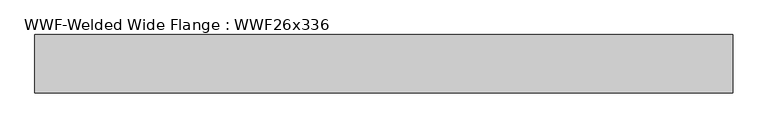
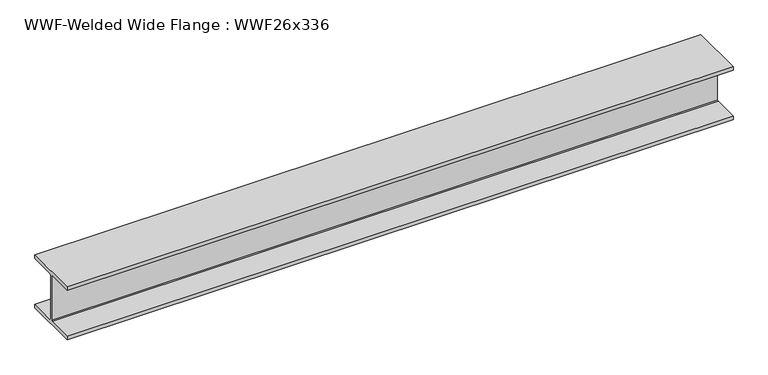
"""IFC4 building model written with IfcOpenShell, lengths in millimetres: beam geometry, WWF-Welded Wide Flange : WWF26x336."""

from ifc_helpers import new_model, si_unit, frame, origin, place, context, project, spatial, polyline, outline, extrude, source, transform, mapped, element, save


def wwf_welded_wide_flange_wwf26x336_1a9bd213(model_context):
    return source(origin(), model_context, "Body", "SweptSolid", [
        extrude(outline(polyline([(324.993, -284.988), (324.993, -324.993), (-324.993, -324.993), (-324.993, -284.988), (-20.6375, -284.988), (-9.9949, -274.3454), (-9.9949, 274.3454), (-20.6375, 284.988), (-324.993, 284.988), (-324.993, 324.993), (324.993, 324.993), (324.993, 284.988), (20.6375, 284.988), (9.9949, 274.3454), (9.9949, -274.3454), (20.6375, -284.988), (324.993, -284.988)])), frame((-3827.7582557, 0.0, 0.0), z_axis=(1.0, 0.0, 0.0), x_axis=(0.0, 1.0, 0.0)), (0.0, 0.0, 1.0), 7762.6459669),
    ])


if __name__ == "__main__":
    model = new_model("IFC4")
    model_context = context("Model", 3, world=origin())
    ifc_project = project(units=[si_unit("LENGTHUNIT", "METRE", prefix="MILLI")], contexts=[model_context])
    site = spatial("IfcSite", under=ifc_project)
    building = spatial("IfcBuilding", under=site)
    placement = place(None, origin())
    wwf_welded_wide_flange_wwf26x336_shape = wwf_welded_wide_flange_wwf26x336_1a9bd213(model_context)
    element("IfcBeam", 1, ObjectType="WWF-Welded Wide Flange : WWF26x336", at=placement, inside=building, context=model_context, shape_type="MappedRepresentation", body=[
        mapped(wwf_welded_wide_flange_wwf26x336_shape, transform((0.0, 0.0, 0.0), x_axis=(1.0, 0.0, 0.0), y_axis=(0.0, 1.0, 0.0), z_axis=(0.0, 0.0, 1.0))),
    ])
    save(model, "model.ifc")

# Revit data of these elements
# Type "WWF-Welded Wide Flange : WWF26x336"
#   Assembly Code = "B10"
#   Nominal d = "12"
#   W = 336
#   Length [instance default] = 1524 mm
#   bf = 649.986 mm
#   d = 649.986 mm
#   k = 20.638 mm
#   tf = 40.005 mm
#   tw = 19.99 mm
#   A = 0.0635483 m²
#   Structural Material [instance default] = Steel ASTM A572
# Element 1 (IfcBeam, "WWF-Welded Wide Flange : WWF26x336")
#   Structural Material = Metal - Steel 43-275
#   Materials on its faces: "Metal - Steel 43-275"
# Materials
#   "Steel ASTM A572": class "Metal", colour RGB 247 247 247, transparency 0, Description = "Structural steel, high strength low alloy, ASTM - A572 - 50", Cost = 0
#   "Metal - Steel 43-275": class "Metal", colour RGB 247 247 247, transparency 0, Cost = 0
